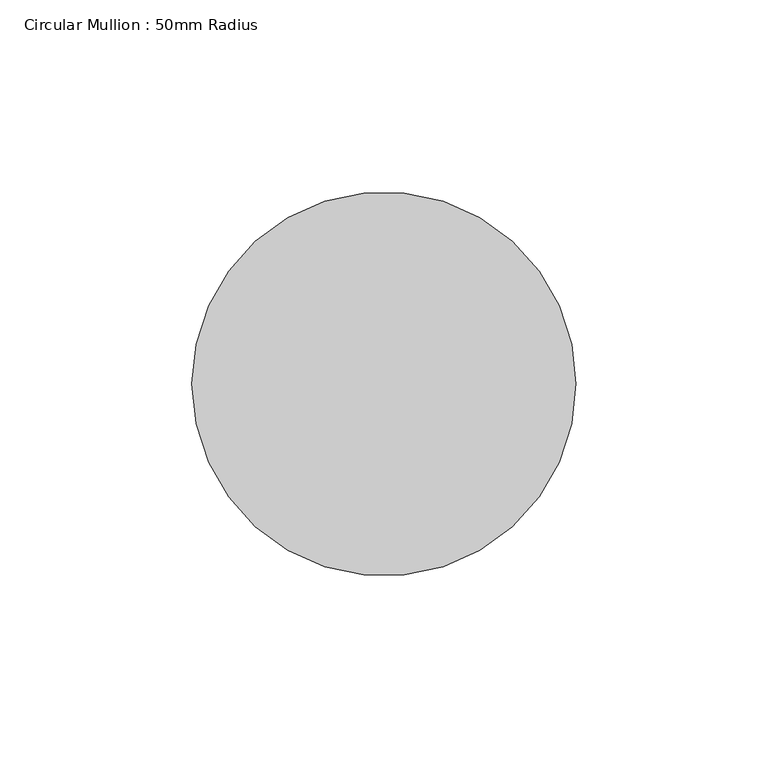
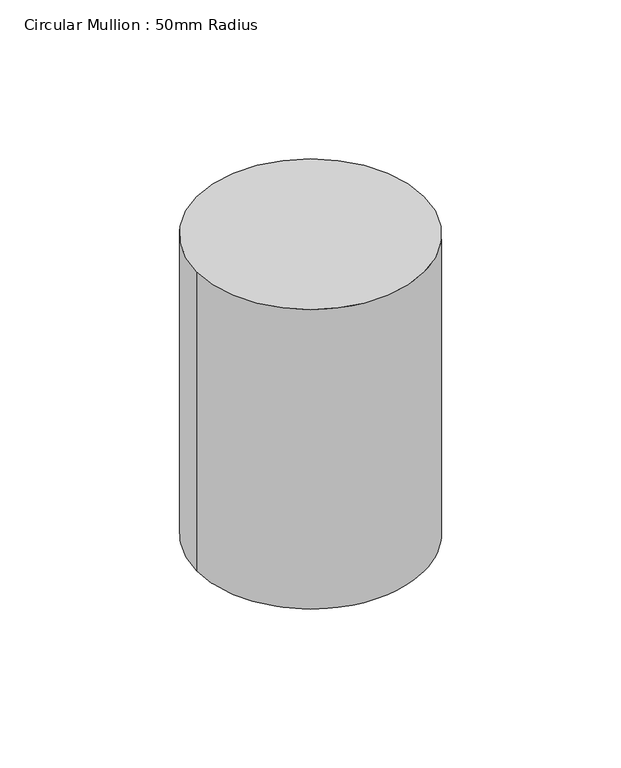
"""IFC4 building model written with IfcOpenShell, lengths in millimetres: member geometry, Circular Mullion : 50mm Radius."""

from ifc_helpers import new_model, si_unit, frame, origin, place, context, project, spatial, circle_curve, ellipse_curve, source, transform, mapped, element, save
from ifc_brep_helpers import plane_surface, cylinder_surface, advanced_brep


def circular_mullion_50mm_radius_48cbdaa6(model_context):
    return source(origin(), model_context, "Body", "AdvancedBrep", [
        advanced_brep(
        [(0.0, 0.0, 0.0), (-100.0, 0.0, 0.0), (0.0, 0.0, -138.6522644), (-100.0, 0.0, -139.0025814)],
        [
            (0, 1, circle_curve(frame((-50.0, 0.0, 0.0), z_axis=(0.0, 0.0, 1.0), x_axis=(1.0, 0.0, 0.0)), 50.0)),
            (1, 0, circle_curve(frame((-50.0, 0.0, 0.0), z_axis=(0.0, 0.0, 1.0), x_axis=(1.0, 0.0, 0.0)), 50.0)),
            (0, 2),
            (2, 3, ellipse_curve(frame((-50.0, 0.0, -138.8274229), z_axis=(-0.003503063038665509, -0.006991464522907234, 0.9999694235191257), x_axis=(0.4479496950727912, 0.8940245626700457, 0.007819976139807781)), 50.0015289, 50.0)),
            (3, 1),
            (3, 2, ellipse_curve(frame((-50.0, 0.0, -138.8274229), z_axis=(-0.003503063038665509, -0.006991464522907234, 0.9999694235191257), x_axis=(0.4479496950727912, 0.8940245626700457, 0.007819976139807781)), 50.0015289, 50.0)),
        ],
        [
            plane_surface(frame((0.0, -100.0, 0.0), z_axis=(0.0, 0.0, 1.0), x_axis=(-1.0, 0.0, 0.0))),
            cylinder_surface(frame((-50.0, 0.0, 0.0), z_axis=(0.0, 0.0, 1.0), x_axis=(1.0, 0.0, 0.0)), 50.0),
            plane_surface(frame((-272.507019, 136.5392419, -138.6522644), z_axis=(0.003503063038665508, 0.0069914645229072325, -0.9999694235191254), x_axis=(0.4479496950727941, 0.8940245626700437, 0.007819976139857134))),
        ],
        [
            (0, [[1, 2]]),
            (1, [[-1, 3, 4, 5]]),
            (1, [[-2, -5, 6, -3]]),
            (2, [[-6, -4]]),
        ],
    ),
    ])


if __name__ == "__main__":
    model = new_model("IFC4")
    model_context = context("Model", 3, world=origin())
    ifc_project = project(units=[si_unit("LENGTHUNIT", "METRE", prefix="MILLI")], contexts=[model_context])
    site = spatial("IfcSite", under=ifc_project)
    building = spatial("IfcBuilding", under=site)
    placement = place(None, origin())
    circular_mullion_50mm_radius_shape = circular_mullion_50mm_radius_48cbdaa6(model_context)
    element("IfcMember", 1, ObjectType="Circular Mullion : 50mm Radius", at=placement, inside=building, context=model_context, shape_type="MappedRepresentation", body=[
        mapped(circular_mullion_50mm_radius_shape, transform((0.0, 0.0, 0.0), x_axis=(1.0, 0.0, 0.0), y_axis=(0.0, 1.0, 0.0), z_axis=(0.0, 0.0, 1.0))),
    ])
    save(model, "model.ifc")

# Revit data of these elements
# Type "Circular Mullion : 50mm Radius"
#   built-in parameter 1007350 = 0.164042 (stored number, unit not read)
# Element 1 (IfcMember, "Circular Mullion : 50mm Radius")
#   Materials on its faces: "Aluminium"
# Materials
#   "Aluminium": class "Metal", colour RGB 247 247 247, transparency 0, Description = "Aluminium 6061", Cost = 0
